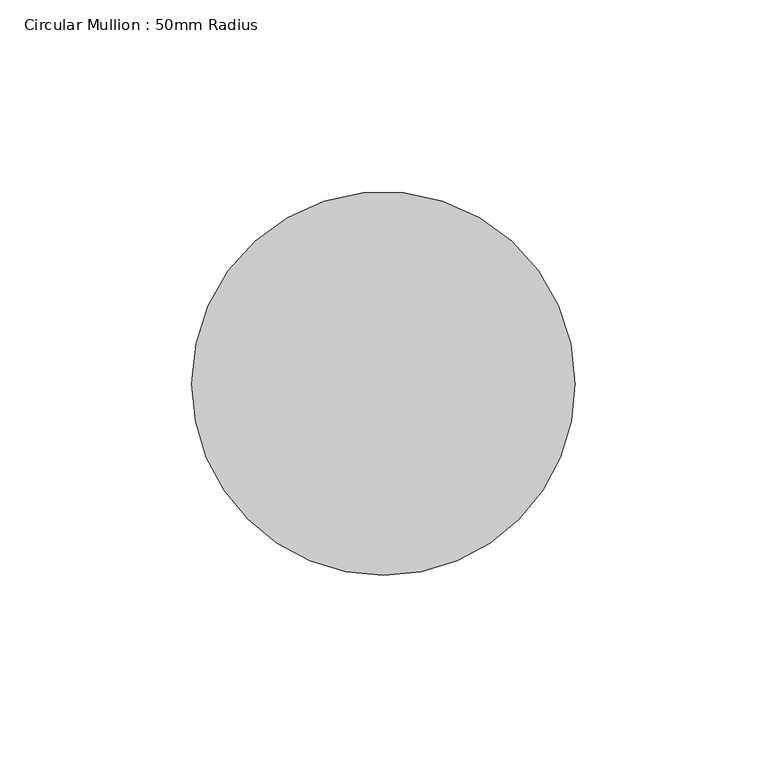
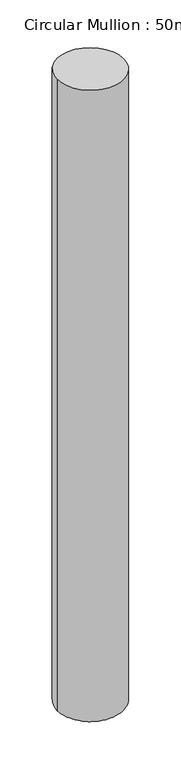
"""IFC4 building model written with IfcOpenShell, lengths in millimetres: member geometry, Circular Mullion : 50mm Radius."""

from ifc_helpers import new_model, si_unit, frame, origin, place, context, project, spatial, ellipse_curve, source, transform, mapped, element, save
from ifc_brep_helpers import plane_surface, cylinder_surface, advanced_brep


def circular_mullion_50mm_radius_ba987735(model_context):
    return source(origin(), model_context, "Body", "AdvancedBrep", [
        advanced_brep(
        [(-100.0, 0.0, 1.7051354), (0.0, 0.0, 0.0), (0.0, 0.0, -1002.215105), (-100.0, 0.0, -1003.9044614)],
        [
            (0, 1, ellipse_curve(frame((-50.0, 0.0, 0.8525677), z_axis=(-0.017047117011896727, -0.01436245902794389, -0.9997515269166902), x_axis=(-0.7645666055457414, -0.6441591583269747, 0.022290904596857068)), 50.0124267, 50.0)),
            (1, 2),
            (2, 3, ellipse_curve(frame((-50.0, 0.0, -1003.0597832), z_axis=(-0.01688944368386278, -0.014229616817022235, 0.9997561026056758), x_axis=(0.7645701048342336, 0.6441621065314691, 0.02208473008006098)), 50.0121978, 50.0)),
            (3, 0),
            (1, 0, ellipse_curve(frame((-50.0, 0.0, 0.8525677), z_axis=(-0.017047117011896727, -0.01436245902794389, -0.9997515269166902), x_axis=(-0.7645666055457414, -0.6441591583269747, 0.022290904596857068)), 50.0124267, 50.0)),
            (3, 2, ellipse_curve(frame((-50.0, 0.0, -1003.0597832), z_axis=(-0.01688944368386278, -0.014229616817022235, 0.9997561026056758), x_axis=(0.7645701048342336, 0.6441621065314691, 0.02208473008006098)), 50.0121978, 50.0)),
        ],
        [
            cylinder_surface(frame((-50.0, 0.0, 0.0), z_axis=(0.0, 0.0, 1.0), x_axis=(1.0, 0.0, 0.0)), 50.0),
            plane_surface(frame((-196.3885087, 233.0978199, 0.0), z_axis=(0.017047117011896727, 0.01436245902794389, 0.9997515269166902), x_axis=(0.7645666055457412, 0.6441591583269748, -0.022290904596867882))),
            plane_surface(frame((-196.3885087, 233.0978199, -1002.215105), z_axis=(0.01688944368386278, 0.014229616817022235, -0.9997561026056758), x_axis=(0.7645701048342336, 0.644162106531469, 0.022084730080072393))),
        ],
        [
            (0, [[1, 2, 3, 4]]),
            (0, [[5, -4, 6, -2]]),
            (1, [[-1, -5]]),
            (2, [[-6, -3]]),
        ],
    ),
    ])


if __name__ == "__main__":
    model = new_model("IFC4")
    model_context = context("Model", 3, world=origin())
    ifc_project = project(units=[si_unit("LENGTHUNIT", "METRE", prefix="MILLI")], contexts=[model_context])
    site = spatial("IfcSite", under=ifc_project)
    building = spatial("IfcBuilding", under=site)
    placement = place(None, origin())
    circular_mullion_50mm_radius_shape = circular_mullion_50mm_radius_ba987735(model_context)
    element("IfcMember", 1, ObjectType="Circular Mullion : 50mm Radius", at=placement, inside=building, context=model_context, shape_type="MappedRepresentation", body=[
        mapped(circular_mullion_50mm_radius_shape, transform((0.0, 0.0, 0.0), x_axis=(1.0, 0.0, 0.0), y_axis=(0.0, 1.0, 0.0), z_axis=(0.0, 0.0, 1.0))),
    ])
    save(model, "model.ifc")

# Revit data of these elements
# Type "Circular Mullion : 50mm Radius"
#   built-in parameter 1007350 = 0.164042 (stored number, unit not read)
# Element 1 (IfcMember, "Circular Mullion : 50mm Radius")
#   Materials on its faces: "Aluminium"
# Materials
#   "Aluminium": class "Metal", colour RGB 247 247 247, transparency 0, Description = "Aluminium 6061", Cost = 0
